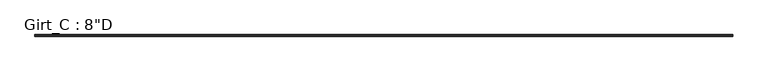
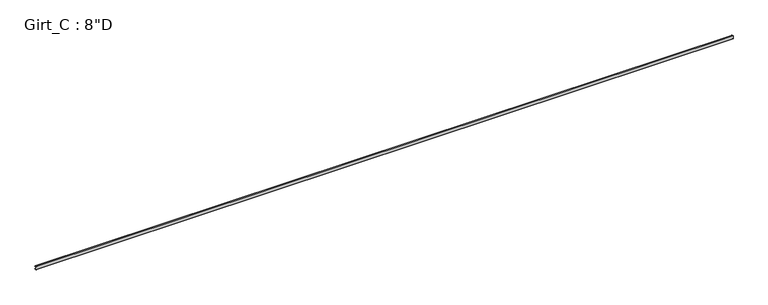
"""IFC4 building model written with IfcOpenShell, lengths in millimetres: beam geometry."""

from ifc_helpers import new_model, si_unit, point, frame, frame_2d, origin, place, context, project, spatial, polyline, circle_curve, trimmed, segment, composite_curve, outline, extrude, source, transform, mapped, element, save


def beam_53796174(model_context):
    return source(origin(), model_context, "Body", "SweptSolid", [
        extrude(outline(composite_curve([segment(polyline([(87.5109375, 101.6), (99.7560415, 87.0068534), (97.6278742, 85.221109), (86.2154765, 98.821875), (3.3005807, 98.821875)]), True, "CONTINUOUS"), segment(trimmed(circle_curve(frame_2d((3.3741066, 96.8381931)), 1.9850441), [point((3.3005807, 98.821875))], [point((1.3890625, 96.8381931))], True, "CARTESIAN"), True, "CONTINUOUS"), segment(polyline([(1.3890625, 96.8381931), (1.3890625, -96.8389339)]), True, "CONTINUOUS"), segment(trimmed(circle_curve(frame_2d((3.3748024, -96.8389339)), 1.9857399), [point((1.3890625, -96.8389339))], [point((3.2694106, -98.821875))], True, "CARTESIAN"), True, "CONTINUOUS"), segment(polyline([(3.2694106, -98.821875), (86.2154765, -98.821875), (97.6510975, -85.1934327), (99.7792647, -86.979177), (87.5109375, -101.6), (3.3734375, -101.6)]), True, "CONTINUOUS"), segment(trimmed(circle_curve(frame_2d((3.3734375, -96.8375)), 4.7625), [point((3.3734375, -101.6))], [point((-1.3890625, -96.8375))], False, "CARTESIAN"), True, "CONTINUOUS"), segment(polyline([(-1.3890625, -96.8375), (-1.3890625, 96.8375)]), True, "CONTINUOUS"), segment(trimmed(circle_curve(frame_2d((3.3734375, 96.8375)), 4.7625), [point((-1.3890625, 96.8375))], [point((3.3734375, 101.6))], False, "CARTESIAN"), True, "CONTINUOUS"), segment(polyline([(3.3734375, 101.6), (87.5109375, 101.6)]), True, "CONTINUOUS")], self_intersect=False)), frame((-22059.9, 0.0, 0.0), z_axis=(1.0, 0.0, 0.0), x_axis=(0.0, 1.0, 0.0)), (0.0, 0.0, 1.0), 44119.8),
    ])


if __name__ == "__main__":
    model = new_model("IFC4")
    model_context = context("Model", 3, world=origin())
    ifc_project = project(units=[si_unit("LENGTHUNIT", "METRE", prefix="MILLI")], contexts=[model_context])
    site = spatial("IfcSite", under=ifc_project)
    building = spatial("IfcBuilding", under=site)
    placement = place(None, origin())
    beam_shape = beam_53796174(model_context)
    element("IfcBeam", 1, ObjectType="Girt_C : 8\"D", at=placement, inside=building, context=model_context, shape_type="MappedRepresentation", body=[
        mapped(beam_shape, transform((0.0, 0.0, 0.0), x_axis=(1.0, 0.0, 0.0), y_axis=(0.0, 1.0, 0.0), z_axis=(0.0, 0.0, 1.0))),
    ])
    save(model, "model.ifc")

# Revit data of these elements
# Type "Girt_C : 8\"D"
#   half leg = 0' - 1 3/4"
#   Web_Thickness = 0' - 0 7/64"
#   Length [instance default] = 10' - 0"
#   Leg_1 = 0' - 3 1/2"
#   Height = 0' - 8"
#   Structural Material [instance default] = none
# Element 1 (IfcBeam, "Girt_C : 8\"D")
#   Materials on its faces: "CEE' SECTION (8.0x3.5C - SEE STRUCT. DWGS)"
# Materials
#   "CEE' SECTION (8.0x3.5C - SEE STRUCT. DWGS)": class "Metal", colour RGB 137 146 153, transparency 0, Description = "Steel, mill finish", Cost = 0
